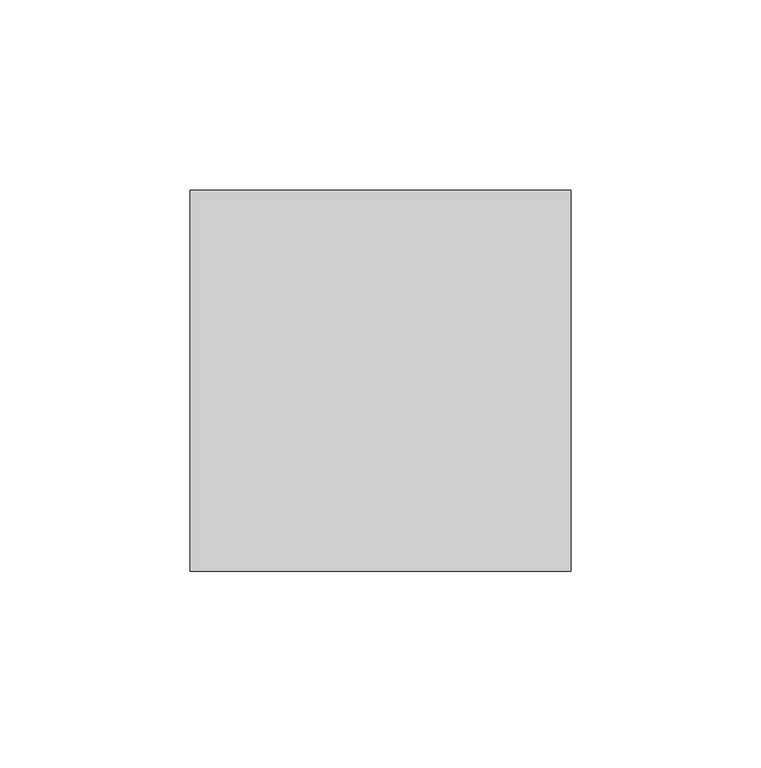
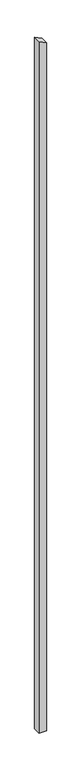
"""IFC4 building model written with IfcOpenShell, lengths in millimetres: column geometry, Holzstütze 158806 : Holzstütze 158806."""

from ifc_helpers import new_model, si_unit, frame, origin, place, context, project, spatial, polyline, outline, extrude, source, transform, mapped, element, save


def column_4e503af9(model_context):
    return source(origin(), model_context, "Body", "SweptSolid", [
        extrude(outline(polyline([(-500.0, 168257.7593015), (-500.0, 168357.7593015), (9372.2929958, 168357.7593015), (9423.2455407, 168257.7593015), (-500.0, 168257.7593015)])), frame((0.0, 47884.7962965, 0.0), z_axis=(0.0, 1.0, 0.0), x_axis=(0.0, 0.0, 1.0)), (0.0, 0.0, 1.0), 100.0),
    ])


if __name__ == "__main__":
    model = new_model("IFC4")
    model_context = context("Model", 3, world=origin())
    ifc_project = project(units=[si_unit("LENGTHUNIT", "METRE", prefix="MILLI")], contexts=[model_context])
    site = spatial("IfcSite", under=ifc_project)
    building = spatial("IfcBuilding", under=site)
    placement = place(None, origin())
    column_shape = column_4e503af9(model_context)
    element("IfcColumn", 1, ObjectType="Holzstütze 158806 : Holzstütze 158806", at=placement, inside=building, context=model_context, shape_type="MappedRepresentation", body=[
        mapped(column_shape, transform((0.0, 0.0, 0.0), x_axis=(1.0, 0.0, 0.0), y_axis=(0.0, 1.0, 0.0), z_axis=(0.0, 0.0, 1.0))),
    ])
    save(model, "model.ifc")

# Revit data of these elements
# Type "Holzstütze 158806 : Holzstütze 158806"
#   Abrechnungsart = "m"
#   Allright_Bauteil_ID = "0152St 0000143380"
#   Bezeichnung = "Holzstütze"
#   Codetext = "ST-HOLZ\\"
#   Gewerk = "Zimmer- und Holzbauarbeiten"
#   Material = "Holz"
#   Objektname = "Stütze"
#   NameOverride = "Holzstütze"
#   Reference = "Holzstütze"
#   Status = "NEW"
#   ThermalTransmittance = 0.0000 BTU/(h·ft²·°F)
#   Roll = 0.00°
#   Slope = 0.00°
#   2D Interaktion = yes
#   IsExternal = yes
#   LoadBearing = yes
# Element 1 (IfcColumn, "Holzstütze 158806 : Holzstütze 158806")
#   Materials on its faces: "holzschalung"
# Materials
#   "holzschalung": class "Unassigned", colour RGB 128 128 128, transparency 0
